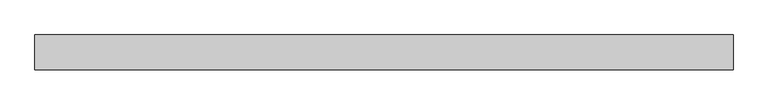
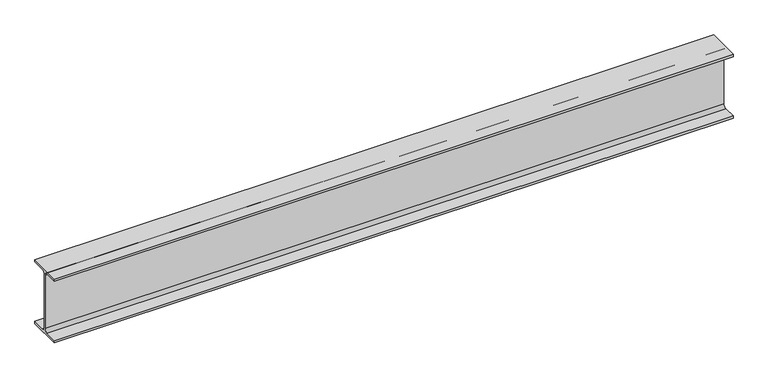
"""IFC4 building model written with IfcOpenShell, lengths in millimetres: beam geometry, 0912_Steel Framing_H-KSD3502 : H_SB_ASB_H-250x125x6x9."""

from ifc_helpers import new_model, si_unit, point, frame, frame_2d, origin, place, context, project, spatial, polyline, circle_curve, trimmed, segment, composite_curve, outline, extrude, source, transform, mapped, element, save


def beam_cc2f091b(model_context):
    return source(origin(), model_context, "Body", "SweptSolid", [
        extrude(outline(composite_curve([segment(polyline([(62.5, -116.0), (62.5, -125.0), (-62.5, -125.0), (-62.5, -116.0), (-15.0, -116.0)]), True, "CONTINUOUS"), segment(trimmed(circle_curve(frame_2d((-15.0, -104.0)), 12.0), [point((-15.0, -116.0))], [point((-3.0, -104.0))], True, "CARTESIAN"), True, "CONTINUOUS"), segment(polyline([(-3.0, -104.0), (-3.0, 104.0)]), True, "CONTINUOUS"), segment(trimmed(circle_curve(frame_2d((-15.0, 104.0)), 12.0), [point((-3.0, 104.0))], [point((-15.0, 116.0))], True, "CARTESIAN"), True, "CONTINUOUS"), segment(polyline([(-15.0, 116.0), (-62.5, 116.0), (-62.5, 125.0), (62.5, 125.0), (62.5, 116.0), (15.0, 116.0)]), True, "CONTINUOUS"), segment(trimmed(circle_curve(frame_2d((15.0, 104.0)), 12.0), [point((15.0, 116.0))], [point((3.0, 104.0))], True, "CARTESIAN"), True, "CONTINUOUS"), segment(polyline([(3.0, 104.0), (3.0, -104.0)]), True, "CONTINUOUS"), segment(trimmed(circle_curve(frame_2d((15.0, -104.0)), 12.0), [point((3.0, -104.0))], [point((15.0, -116.0))], True, "CARTESIAN"), True, "CONTINUOUS"), segment(polyline([(15.0, -116.0), (62.5, -116.0)]), True, "CONTINUOUS")], self_intersect=False)), frame((-1337.3, 0.0, 0.0), z_axis=(1.0, 0.0, 0.0), x_axis=(0.0, 1.0, 0.0)), (0.0, 0.0, 1.0), 2511.6),
    ])


if __name__ == "__main__":
    model = new_model("IFC4")
    model_context = context("Model", 3, world=origin())
    ifc_project = project(units=[si_unit("LENGTHUNIT", "METRE", prefix="MILLI")], contexts=[model_context])
    site = spatial("IfcSite", under=ifc_project)
    building = spatial("IfcBuilding", under=site)
    placement = place(None, origin())
    beam_shape = beam_cc2f091b(model_context)
    element("IfcBeam", 1, ObjectType="0912_Steel Framing_H-KSD3502 : H_SB_ASB_H-250x125x6x9", at=placement, inside=building, context=model_context, shape_type="MappedRepresentation", body=[
        mapped(beam_shape, transform((0.0, 0.0, 0.0), x_axis=(1.0, 0.0, 0.0), y_axis=(0.0, 1.0, 0.0), z_axis=(0.0, 0.0, 1.0))),
    ])
    save(model, "model.ifc")

# Revit data of these elements
# Type "0912_Steel Framing_H-KSD3502 : H_SB_ASB_H-250x125x6x9"
#   H_WM Code_1 = "S01AA003-00001 | Main Steel Structure Fabrication Work | Shelter/Building | Light Steel - Standard (30KG/M>Weight) | Material: (   )"
#   H_WM Code_2 = "S03AA029-00001 | Main Steel Structure Erection Work | Shelter/Building | Light Steel (30KG/M>Weight) | Material: (   )"
#   H_WM Code_3 = "S01AA010-00001 | Main Steel Structure Fabrication Work | Shelter/Building | Steel Painting/Coating | for Non-Fireproofed Steel Surface, Surface Preparation, Primer, Second & Final Coat | Material: (   )"
#   H_Q'ty Cal Type Tag = "SB-Q2"
#   Width = 12.5 cm
#   Web Thickness = 0.6 cm
#   Web Fillet = 1.2 cm
#   Warping Constant = 42539.8 cm⁶
#   W = 0
#   Torsional Moment of Inertia = 7.8102 cm⁴
#   Section Area = 37.66 cm²
#   Plastic Modulus weak axis = 73.1 cm³
#   Plastic Modulus strong axis = 366.0 cm³
#   Perimeter = 0.97 m²/m
#   Nominal Weight = 29.60 kgf/m
#   Moment of Inertia weak axis = 294.00 cm⁴
#   Moment of Inertia strong axis = 4050.00 cm⁴
#   Height = 25.0 cm
#   Flange Thickness = 0.9 cm
#   Elastic Modulus weak axis = 47.0 cm³
#   Elastic Modulus strong axis = 324.0 cm³
#   Centroid Vertical = 12.5 cm
#   Centroid Horizontal = 6.25 cm
#   Ix = 40500000
#   Length [instance default] = 1.5240 m
#   Zx = 366000
#   b = 0.1250 m
#   h = 0.2500 m
#   r = 0.0120 m
#   s = 0.0060 m
#   t = 0.0090 m
#   A = 0.003766 m²
#   Structural Material [instance default] = Steel, 45-345
#   Assembly Code = ""
# Element 1 (IfcBeam, "0912_Steel Framing_H-KSD3502 : H_SB_ASB_H-250x125x6x9")
#   Structural Material = none
# Materials
#   "Steel, 45-345": class "Metal", colour RGB 189 187 185, transparency 0, Description = "Steel 345 MPa", Cost = 0
